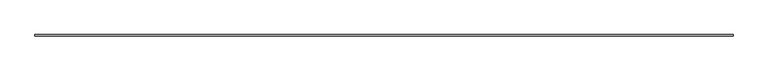
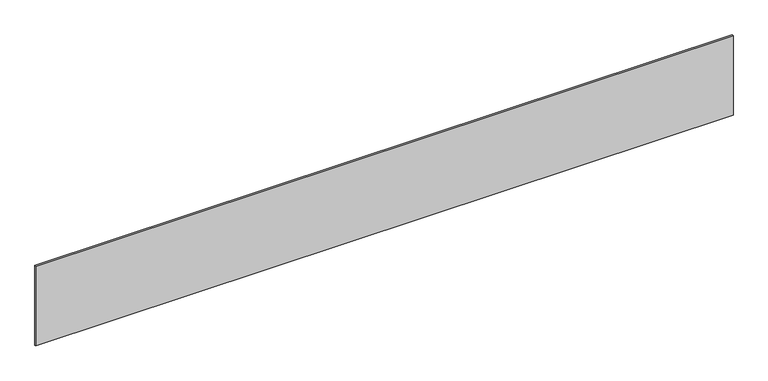
"""IFC4 building model written with IfcOpenShell, lengths in millimetres: proxy geometry, Inner panel:Inner panel:1:Inner panel:1 : Inner panel:Inner panel:300324:300043:Inner panel:1:Inner panel:1 : Inner panel:Inner panel:300324:300043 : Inner panel:Inner panel:1:Inner panel:1 : Inner panel:Inner panel:300324:300043:37 : Inner panel:Inner panel:1:Inner panel:1 : Inner panel:Inner panel:300324:300043:Inner panel:1:Inner panel:1 : Inner panel:Inner panel:300324:300043 : Inner panel:Inner panel:1:Inner panel:1 : Inner panel:Inner panel:300324:300043:300031."""

from ifc_helpers import new_model, si_unit, frame, origin, place, context, project, spatial, polyline, outline, extrude, source, transform, mapped, element, save


def generic_models_6ef6e33d(model_context):
    return source(origin(), model_context, "Body", "SweptSolid", [
        extrude(outline(polyline([(560365.6617239, -578778.4413841), (570446.2867239, -578778.4413841), (570446.2867239, -578797.4913841), (560365.6617239, -578797.4913841), (560365.6617239, -578778.4413841)])), frame((0.0, 0.0, 3721.1), z_axis=(0.0, 0.0, 1.0), x_axis=(1.0, 0.0, 0.0)), (0.0, 0.0, 1.0), 1219.2),
    ])


if __name__ == "__main__":
    model = new_model("IFC4")
    model_context = context("Model", 3, world=origin())
    ifc_project = project(units=[si_unit("LENGTHUNIT", "METRE", prefix="MILLI")], contexts=[model_context])
    site = spatial("IfcSite", under=ifc_project)
    building = spatial("IfcBuilding", under=site)
    placement = place(None, origin())
    generic_models_shape = generic_models_6ef6e33d(model_context)
    element("IfcBuildingElementProxy", 1, Name="Inner panel:Inner panel:1:Inner panel:1 : Inner panel:Inner panel:300324:300043:Inner panel:1:Inner panel:1 : Inner panel:Inner panel:300324:300043 : Inner panel:Inner panel:1:Inner panel:1 : Inner panel:Inner panel:300324:300043:37 : Inner panel:Inner panel:1:Inner panel:1 : Inner panel:Inner panel:300324:300043:Inner panel:1:Inner panel:1 : Inner panel:Inner panel:300324:300043 : Inner panel:Inner panel:1:Inner panel:1 : Inner panel:Inner panel:300324:300043:300031", ObjectType="Inner panel:Inner panel:1:Inner panel:1 : Inner panel:Inner panel:300324:300043:Inner panel:1:Inner panel:1 : Inner panel:Inner panel:300324:300043 : Inner panel:Inner panel:1:Inner panel:1 : Inner panel:Inner panel:300324:300043:37 : Inner panel:Inner panel:1:Inner panel:1 : Inner panel:Inner panel:300324:300043:Inner panel:1:Inner panel:1 : Inner panel:Inner panel:300324:300043 : Inner panel:Inner panel:1:Inner panel:1 : Inner panel:Inner panel:300324:300043:300031", at=placement, inside=building, context=model_context, shape_type="MappedRepresentation", body=[
        mapped(generic_models_shape, transform((0.0, 0.0, 0.0), x_axis=(1.0, 0.0, 0.0), y_axis=(0.0, 1.0, 0.0), z_axis=(0.0, 0.0, 1.0))),
    ])
    save(model, "model.ifc")

# Revit data of these elements
# Type "Inner panel:Inner panel:1:Inner panel:1 : Inner panel:Inner panel:300324:300043:Inner panel:1:Inner panel:1 : Inner panel:Inner panel:300324:300043 : Inner panel:Inner panel:1:Inner panel:1 : Inner panel:Inner panel:300324:300043:37 : Inner panel:Inner panel:1:Inner panel:1 : Inner panel:Inner panel:300324:300043:Inner panel:1:Inner panel:1 : Inner panel:Inner panel:300324:300043 : Inner panel:Inner panel:1:Inner panel:1 : Inner panel:Inner panel:300324:300043:300031"
#   NameOverride = "Inner panel:Inner panel:1:Inner panel:1 : Inner panel:Inner panel:300324:300043:Inner panel:1:Inner panel:1 : Inner panel:Inner panel:300324:300043 : Inner panel:Inner panel:1:Inner panel:1 : Inner panel:Inner panel:300324:300043:300031"
#   ObjectTypeOverride = "Inner panel:1:Inner panel:1 : Inner panel:Inner panel:300324:300043 : Inner panel:Inner panel:1:Inner panel:1 : Inner panel:Inner panel:300324:300043"
#   Reference = "Inner panel"
#   Tag = "300031"
# Element 1 (IfcBuildingElementProxy, "Inner panel:Inner panel:1:Inner panel:1 : Inner panel:Inner panel:300324:300043:Inner panel:1:Inner panel:1 : Inner panel:Inner panel:300324:300043 : Inner panel:Inner panel:1:Inner panel:1 : Inner panel:Inner panel:300324:300043:37 : Inner panel:Inner panel:1:Inner panel:1 : Inner panel:Inner panel:300324:300043:Inner panel:1:Inner panel:1 : Inner panel:Inner panel:300324:300043 : Inner panel:Inner panel:1:Inner panel:1 : Inner panel:Inner panel:300324:300043:300031")
#   Materials on its faces: "3/4\" EXTERIOR GRADE FIRE RETARDANT PLYWOOD (FINISH: GRADE B)"
# Materials
#   "3/4\" EXTERIOR GRADE FIRE RETARDANT PLYWOOD (FINISH: GRADE B)": class "Wood", colour RGB 149 120 74, transparency 0, Description = "Plywood, sheathing grade", Cost = 0
